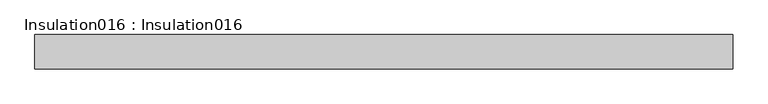
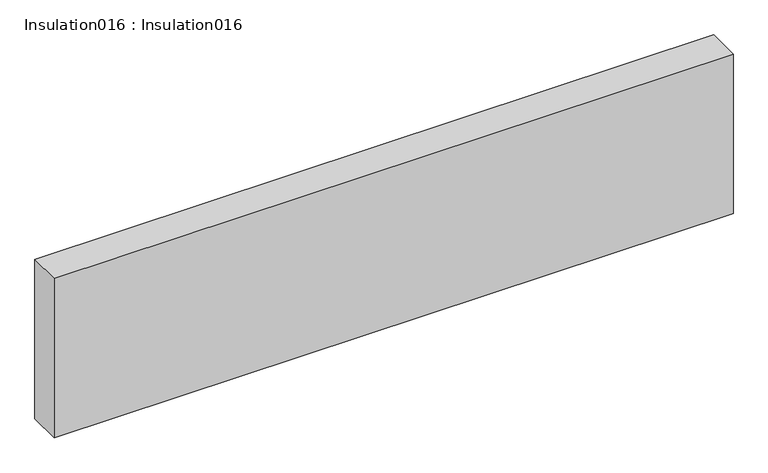
"""IFC4 building model written with IfcOpenShell, lengths in millimetres: proxy geometry, Insulation016 : Insulation016."""

from ifc_helpers import new_model, si_unit, frame, origin, place, context, project, spatial, polyline, outline, extrude, source, transform, mapped, element, save


def insulation016_insulation016_28f28b75(model_context):
    return source(origin(), model_context, "Body", "SweptSolid", [
        extrude(outline(polyline([(12383.0178845, -4623.3864821), (12383.0178845, -4524.9614258), (14383.0178845, -4524.9614258), (14383.0178845, -4623.3864821), (12383.0178845, -4623.3864821)])), frame((0.0, 0.0, 39158.7959974), z_axis=(0.0, 0.0, 1.0), x_axis=(1.0, 0.0, 0.0)), (0.0, 0.0, 1.0), 496.7000026),
    ])


if __name__ == "__main__":
    model = new_model("IFC4")
    model_context = context("Model", 3, world=origin())
    ifc_project = project(units=[si_unit("LENGTHUNIT", "METRE", prefix="MILLI")], contexts=[model_context])
    site = spatial("IfcSite", under=ifc_project)
    building = spatial("IfcBuilding", under=site)
    placement = place(None, origin())
    insulation016_insulation016_shape = insulation016_insulation016_28f28b75(model_context)
    element("IfcBuildingElementProxy", 1, Name="Insulation016 : Insulation016", ObjectType="Insulation016 : Insulation016", at=placement, inside=building, context=model_context, shape_type="MappedRepresentation", body=[
        mapped(insulation016_insulation016_shape, transform((0.0, 0.0, 0.0), x_axis=(1.0, 0.0, 0.0), y_axis=(0.0, 1.0, 0.0), z_axis=(0.0, 0.0, 1.0))),
    ])
    save(model, "model.ifc")

# Revit data of these elements
# Type "Insulation016 : Insulation016"
#   NameOverride = "Insulation016"
# Element 1 (IfcBuildingElementProxy, "Insulation016 : Insulation016")
#   Materials on its faces: "BATT INSULATION (U-FACTOR = 0.065 MIN.) OVER CLASS II VAPOR RETARDER (TOWARDS INTERIOR)"
# Materials
#   "BATT INSULATION (U-FACTOR = 0.065 MIN.) OVER CLASS II VAPOR RETARDER (TOWARDS INTERIOR)": class "Unassigned", colour RGB 246 242 160, transparency 0, Cost = 0
